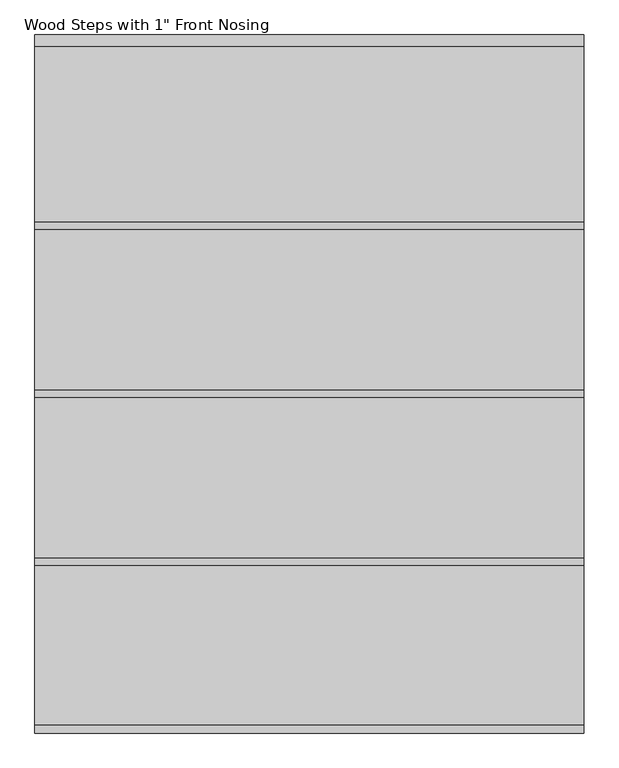
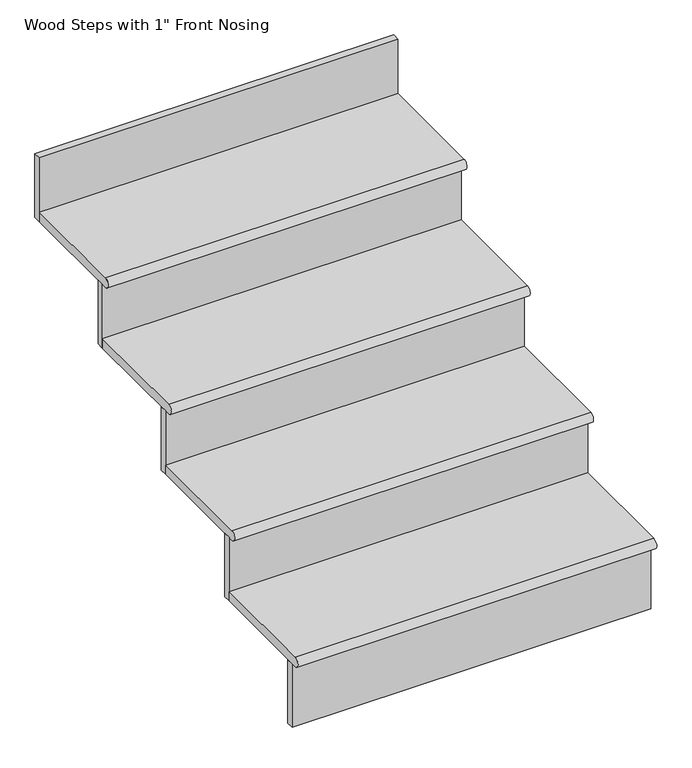
"""IFC4 building model written with IfcOpenShell, lengths in millimetres: stair flight geometry."""

from ifc_helpers import new_model, si_unit, point, frame, frame_2d, origin, place, context, project, spatial, polyline, circle_curve, trimmed, segment, composite_curve, outline, extrude, source, transform, mapped, element, save


def stair_flight_9f9bb81b(model_context):
    return source(origin(), model_context, "Body", "SweptSolid", [
        extrude(outline(composite_curve([segment(polyline([(-12436.2557429, 1885.95), (-12144.1557429, 1885.95), (-12144.1557429, 1860.55), (-12436.2557429, 1860.55)]), True, "CONTINUOUS"), segment(trimmed(circle_curve(frame_2d((-12436.2557429, 1873.25)), 12.7), [point((-12436.2557429, 1860.55))], [point((-12436.2557429, 1885.95))], False, "CARTESIAN"), True, "CONTINUOUS")], self_intersect=False)), frame((6489.8789345, 0.0, 0.0), z_axis=(1.0, 0.0, 0.0), x_axis=(0.0, 1.0, 0.0)), (0.0, 0.0, 1.0), 914.4),
        extrude(outline(polyline([(7404.2789345, -12404.5057429), (7404.2789345, -12423.5557429), (6489.8789345, -12423.5557429), (6489.8789345, -12404.5057429), (7404.2789345, -12404.5057429)])), frame((0.0, 0.0, 1689.1), z_axis=(0.0, 0.0, 1.0), x_axis=(1.0, 0.0, 0.0)), (0.0, 0.0, 1.0), 171.45),
        extrude(outline(polyline([(7404.2789345, -12125.1057429), (7404.2789345, -12144.1557429), (6489.8789345, -12144.1557429), (6489.8789345, -12125.1057429), (7404.2789345, -12125.1057429)])), frame((0.0, 0.0, 1860.55), z_axis=(0.0, 0.0, 1.0), x_axis=(1.0, 0.0, 0.0)), (0.0, 0.0, 1.0), 171.45),
        extrude(outline(composite_curve([segment(polyline([(-12156.8557429, 2057.4), (-11864.7557429, 2057.4), (-11864.7557429, 2032.0), (-12156.8557429, 2032.0)]), True, "CONTINUOUS"), segment(trimmed(circle_curve(frame_2d((-12156.8557429, 2044.7)), 12.7), [point((-12156.8557429, 2032.0))], [point((-12156.8557429, 2057.4))], False, "CARTESIAN"), True, "CONTINUOUS")], self_intersect=False)), frame((6489.8789345, 0.0, 0.0), z_axis=(1.0, 0.0, 0.0), x_axis=(0.0, 1.0, 0.0)), (0.0, 0.0, 1.0), 914.4),
        extrude(outline(polyline([(7404.2789345, -11845.7057429), (7404.2789345, -11864.7557429), (6489.8789345, -11864.7557429), (6489.8789345, -11845.7057429), (7404.2789345, -11845.7057429)])), frame((0.0, 0.0, 2032.0), z_axis=(0.0, 0.0, 1.0), x_axis=(1.0, 0.0, 0.0)), (0.0, 0.0, 1.0), 171.45),
        extrude(outline(composite_curve([segment(polyline([(-11877.4557429, 2228.85), (-11585.3557429, 2228.85), (-11585.3557429, 2203.45), (-11877.4557429, 2203.45)]), True, "CONTINUOUS"), segment(trimmed(circle_curve(frame_2d((-11877.4557429, 2216.15)), 12.7), [point((-11877.4557429, 2203.45))], [point((-11877.4557429, 2228.85))], False, "CARTESIAN"), True, "CONTINUOUS")], self_intersect=False)), frame((6489.8789345, 0.0, 0.0), z_axis=(1.0, 0.0, 0.0), x_axis=(0.0, 1.0, 0.0)), (0.0, 0.0, 1.0), 914.4),
        extrude(outline(polyline([(7404.2789345, -11566.3057429), (7404.2789345, -11585.3557429), (6489.8789345, -11585.3557429), (6489.8789345, -11566.3057429), (7404.2789345, -11566.3057429)])), frame((0.0, 0.0, 2203.45), z_axis=(0.0, 0.0, 1.0), x_axis=(1.0, 0.0, 0.0)), (0.0, 0.0, 1.0), 171.45),
        extrude(outline(polyline([(7404.2789345, -11286.9057429), (7404.2789345, -11305.9557429), (6489.8789345, -11305.9557429), (6489.8789345, -11286.9057429), (7404.2789345, -11286.9057429)])), frame((0.0, 0.0, 2374.9), z_axis=(0.0, 0.0, 1.0), x_axis=(1.0, 0.0, 0.0)), (0.0, 0.0, 1.0), 171.45),
        extrude(outline(composite_curve([segment(polyline([(-11598.0557429, 2400.3), (-11305.9557429, 2400.3), (-11305.9557429, 2374.9), (-11598.0557429, 2374.9)]), True, "CONTINUOUS"), segment(trimmed(circle_curve(frame_2d((-11598.0557429, 2387.6)), 12.7), [point((-11598.0557429, 2374.9))], [point((-11598.0557429, 2400.3))], False, "CARTESIAN"), True, "CONTINUOUS")], self_intersect=False)), frame((6489.8789345, 0.0, 0.0), z_axis=(1.0, 0.0, 0.0), x_axis=(0.0, 1.0, 0.0)), (0.0, 0.0, 1.0), 914.4),
    ])


if __name__ == "__main__":
    model = new_model("IFC4")
    model_context = context("Model", 3, world=origin())
    ifc_project = project(units=[si_unit("LENGTHUNIT", "METRE", prefix="MILLI")], contexts=[model_context])
    site = spatial("IfcSite", under=ifc_project)
    building = spatial("IfcBuilding", under=site)
    placement = place(None, origin())
    stair_flight_shape = stair_flight_9f9bb81b(model_context)
    element("IfcStairFlight", 1, ObjectType="Wood Steps with 1\" Front Nosing", at=placement, inside=building, context=model_context, shape_type="MappedRepresentation", body=[
        mapped(stair_flight_shape, transform((0.0, 0.0, 0.0), x_axis=(1.0, 0.0, 0.0), y_axis=(0.0, 1.0, 0.0), z_axis=(0.0, 0.0, 1.0))),
    ])
    save(model, "model.ifc")

# Revit data of these elements
# Element 1 (IfcStairFlight, "Wood Steps with 1\" Front Nosing")
#   Materials on its faces: "Paints and Coatings", "Cherry"
# Materials
#   "Paints and Coatings": class "Paint", colour RGB 244 244 244, transparency 0, Description = "Interior finish", Cost = 0
#   "Cherry": class "Wood", colour RGB 233 182 144, transparency 0, Description = "Prunus Serotina", Cost = 0
